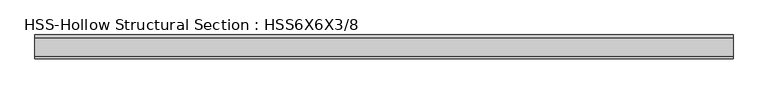
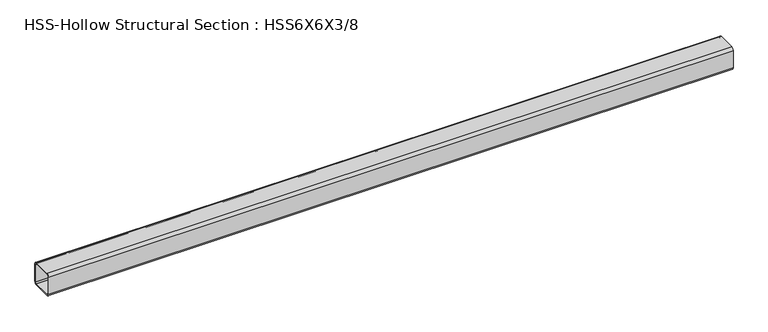
"""IFC4 building model written with IfcOpenShell, lengths in millimetres: member geometry, HSS-Hollow Structural Section : HSS6X6X3/8."""

from ifc_helpers import new_model, si_unit, point, frame, frame_2d, origin, place, context, project, spatial, polyline, circle_curve, trimmed, segment, composite_curve, outline, extrude, source, transform, mapped, element, save


def hss_hollow_structural_section_hss6x6x3_8_4cd37dbb(model_context):
    return source(origin(), model_context, "Body", "SweptSolid", [
        extrude(outline(composite_curve([segment(polyline([(76.2, 58.4708), (76.2, -58.4708)]), True, "CONTINUOUS"), segment(trimmed(circle_curve(frame_2d((58.4708, -58.4708)), 17.7292), [point((76.2, -58.4708))], [point((58.4708, -76.2))], False, "CARTESIAN"), True, "CONTINUOUS"), segment(polyline([(58.4708, -76.2), (-58.4708, -76.2)]), True, "CONTINUOUS"), segment(trimmed(circle_curve(frame_2d((-58.4708, -58.4708)), 17.7292), [point((-58.4708, -76.2))], [point((-76.2, -58.4708))], False, "CARTESIAN"), True, "CONTINUOUS"), segment(polyline([(-76.2, -58.4708), (-76.2, 58.4708)]), True, "CONTINUOUS"), segment(trimmed(circle_curve(frame_2d((-58.4708, 58.4708)), 17.7292), [point((-76.2, 58.4708))], [point((-58.4708, 76.2))], False, "CARTESIAN"), True, "CONTINUOUS"), segment(polyline([(-58.4708, 76.2), (58.4708, 76.2)]), True, "CONTINUOUS"), segment(trimmed(circle_curve(frame_2d((58.4708, 58.4708)), 17.7292), [point((58.4708, 76.2))], [point((76.2, 58.4708))], False, "CARTESIAN"), True, "CONTINUOUS")], self_intersect=False), holes=[composite_curve([segment(trimmed(circle_curve(frame_2d((-58.4708, 58.4708)), 8.8646), [point((-58.4708, 67.3354))], [point((-67.3354, 58.4708))], True, "CARTESIAN"), True, "CONTINUOUS"), segment(polyline([(-67.3354, 58.4708), (-67.3354, -58.4708)]), True, "CONTINUOUS"), segment(trimmed(circle_curve(frame_2d((-58.4708, -58.4708)), 8.8646), [point((-67.3354, -58.4708))], [point((-58.4708, -67.3354))], True, "CARTESIAN"), True, "CONTINUOUS"), segment(polyline([(-58.4708, -67.3354), (58.4708, -67.3354)]), True, "CONTINUOUS"), segment(trimmed(circle_curve(frame_2d((58.4708, -58.4708)), 8.8646), [point((58.4708, -67.3354))], [point((67.3354, -58.4708))], True, "CARTESIAN"), True, "CONTINUOUS"), segment(polyline([(67.3354, -58.4708), (67.3354, 58.4708)]), True, "CONTINUOUS"), segment(trimmed(circle_curve(frame_2d((58.4708, 58.4708)), 8.8646), [point((67.3354, 58.4708))], [point((58.4708, 67.3354))], True, "CARTESIAN"), True, "CONTINUOUS"), segment(polyline([(58.4708, 67.3354), (-58.4708, 67.3354)]), True, "CONTINUOUS")], self_intersect=False)]), frame((-2238.0009497, 0.0, 0.0), z_axis=(1.0, 0.0, 0.0), x_axis=(0.0, 1.0, 0.0)), (0.0, 0.0, 1.0), 4449.0151793),
    ])


if __name__ == "__main__":
    model = new_model("IFC4")
    model_context = context("Model", 3, world=origin())
    ifc_project = project(units=[si_unit("LENGTHUNIT", "METRE", prefix="MILLI")], contexts=[model_context])
    site = spatial("IfcSite", under=ifc_project)
    building = spatial("IfcBuilding", under=site)
    placement = place(None, origin())
    hss_hollow_structural_section_hss6x6x3_8_shape = hss_hollow_structural_section_hss6x6x3_8_4cd37dbb(model_context)
    element("IfcMember", 1, ObjectType="HSS-Hollow Structural Section : HSS6X6X3/8", at=placement, inside=building, context=model_context, shape_type="MappedRepresentation", body=[
        mapped(hss_hollow_structural_section_hss6x6x3_8_shape, transform((0.0, 0.0, 0.0), x_axis=(1.0, 0.0, 0.0), y_axis=(0.0, 1.0, 0.0), z_axis=(0.0, 0.0, 1.0))),
    ])
    save(model, "model.ifc")

# Revit data of these elements
# Type "HSS-Hollow Structural Section : HSS6X6X3/8"
#   Assembly Code = "B10"
#   Shape = "Square"
#   W = 27.4
#   Ht = 0' - 6"
#   Length [instance default] = 5' - 0"
#   b = 0' - 6"
#   kr = 0' - 0.698"
#   t = 0' - 0.349"
#   A = 0.0526389 SF
#   Structural Material [instance default] = Steel ASTM A500, Grade B, Rectangular and Square
# Element 1 (IfcMember, "HSS-Hollow Structural Section : HSS6X6X3/8")
#   Materials on its faces: "Steel ASTM A500, Grade B, Rectangular and Square"
# Materials
#   "Steel ASTM A500, Grade B, Rectangular and Square": class "Metal", colour RGB 199 199 199, transparency 0, Description = "Carbon steel", Cost = 0
